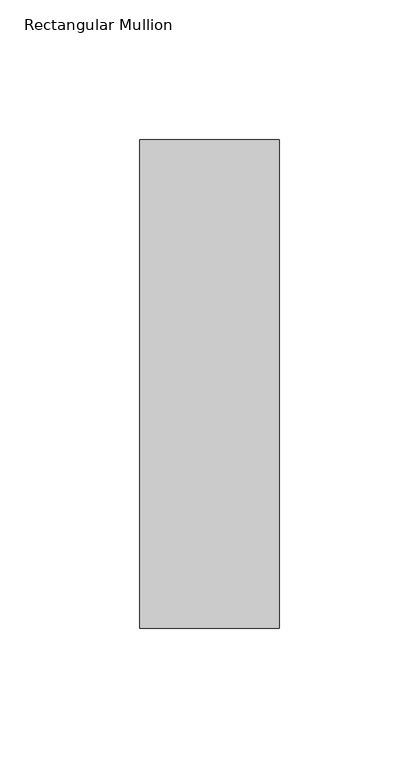
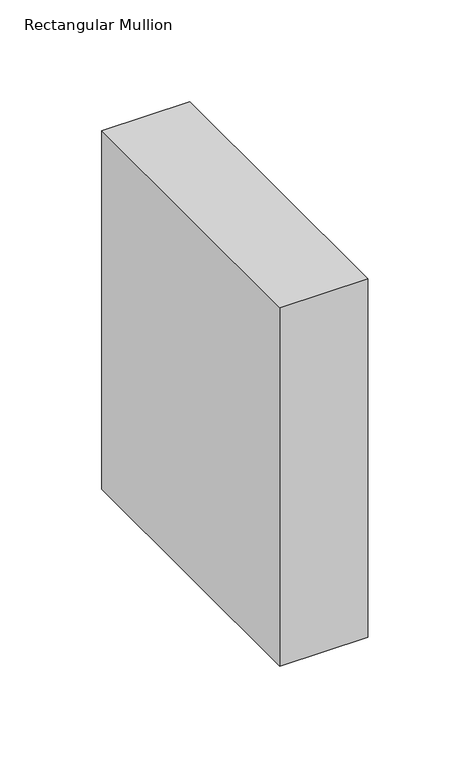
"""IFC4 building model written with IfcOpenShell, lengths in millimetres: member geometry, Rectangular Mullion : WWm-50x175-50mmOffset."""

import ifcopenshell
import ifcopenshell.guid

model = None  # the IFC model being written
_history = None  # IfcOwnerHistory: only IFC2X3 demands one
_inside = {}  # id of a spatial element -> (the spatial element, [elements in it])
_under = {}  # id of a project, library or spatial element -> (it, [spatial elements below it])
_declared = {}  # id of a project -> (the project, [libraries it declares])
_typed = {}  # id of a type object -> (the type object, [elements of that type])
_made_of = {}  # id of a material, layer set ... -> (it, [elements and type objects made of it])


def new_model(schema):
    """Start an empty IFC model of exactly this schema.

    Asked for "IFC4X3", IfcOpenShell would pick the latest addendum, in which some entities
    have other attributes; the version numbers below select the first issue.
    IFC2X3 requires an IfcOwnerHistory on every rooted entity: one is made here for all.
    """
    global model, _history
    if schema == "IFC4X3":
        model = ifcopenshell.file(schema_version=(4, 3, 0, 0))
    else:
        model = ifcopenshell.file(schema=schema)
    _inside.clear()
    _under.clear()
    _declared.clear()
    _typed.clear()
    _made_of.clear()
    _history = None
    if model.schema == "IFC2X3":
        org = make("IfcOrganization", Name="unknown")
        user = make(
            "IfcPersonAndOrganization",
            ThePerson=make("IfcPerson", FamilyName="unknown"),
            TheOrganization=org,
        )
        app = make(
            "IfcApplication",
            ApplicationDeveloper=org,
            Version="unknown",
            ApplicationFullName="unknown",
            ApplicationIdentifier="unknown",
        )
        _history = make(
            "IfcOwnerHistory",
            OwningUser=user,
            OwningApplication=app,
            ChangeAction="ADDED",
            CreationDate=0,
        )
    return model


def make(cls, **values):
    """One entity of the class cls with the attributes given. An attribute that is None is left unset."""
    return model.create_entity(
        cls, **{name: value for name, value in values.items() if value is not None}
    )


def rooted(cls, **values):
    """An entity with a GlobalId (a new one), such as an element, a storey or a relation."""
    return make(cls, GlobalId=ifcopenshell.guid.new(), OwnerHistory=_history, **values)


def si_unit(unit_type, name, prefix=None):
    """IfcSIUnit, for example si_unit("LENGTHUNIT", "METRE", prefix="MILLI")."""
    return make("IfcSIUnit", UnitType=unit_type, Prefix=prefix, Name=name)


def assignment(units):
    """IfcUnitAssignment: the units of a project."""
    return None if units is None else make("IfcUnitAssignment", Units=units)


def point(xyz):
    """IfcCartesianPoint."""
    return None if xyz is None else make("IfcCartesianPoint", Coordinates=xyz)


def direction(xyz):
    """IfcDirection."""
    return None if xyz is None else make("IfcDirection", DirectionRatios=xyz)


def frame(location, z_axis=None, x_axis=None):
    """IfcAxis2Placement3D, a coordinate frame: its origin and axes. An axis left out is left unset."""
    return make(
        "IfcAxis2Placement3D",
        Location=point(location),
        Axis=direction(z_axis),
        RefDirection=direction(x_axis),
    )


def origin():
    """The frame at (0, 0, 0) with its axes left unset."""
    return frame((0.0, 0.0, 0.0))


def place(relative_to, where):
    """IfcLocalPlacement: puts the frame where relative to a parent placement (None: the world)."""
    return make(
        "IfcLocalPlacement", PlacementRelTo=relative_to, RelativePlacement=where
    )


def context(
    kind, dimensions, precision=None, world=None, true_north=None, identifier=None
):
    """IfcGeometricRepresentationContext, for example the 3D "Model" context."""
    return make(
        "IfcGeometricRepresentationContext",
        ContextIdentifier=identifier,
        ContextType=kind,
        CoordinateSpaceDimension=dimensions,
        Precision=precision,
        WorldCoordinateSystem=world,
        TrueNorth=true_north,
    )


def project(units=None, contexts=None):
    """IfcProject with its units and contexts."""
    return rooted(
        "IfcProject",
        Name="project",
        RepresentationContexts=contexts,
        UnitsInContext=assignment(units),
    )


def spatial(cls, under=None, at=None, **own):
    """A site, building, storey or space (cls), placed at a placement, below another one or the project."""
    s = rooted(cls, ObjectPlacement=at, **own)
    if under is not None:
        _under.setdefault(under.id(), (under, []))[1].append(s)
    return s


def polyline(points):
    """IfcPolyline through the points."""
    return make("IfcPolyline", Points=[point(p) for p in points])


def outline(outer, holes=None, kind="AREA"):
    """IfcArbitraryClosedProfileDef: a profile drawn as a closed curve; with holes, ...WithVoids."""
    if holes is None:
        return make("IfcArbitraryClosedProfileDef", ProfileType=kind, OuterCurve=outer)
    return make(
        "IfcArbitraryProfileDefWithVoids",
        ProfileType=kind,
        OuterCurve=outer,
        InnerCurves=holes,
    )


def extrude(swept, where, along, depth):
    """IfcExtrudedAreaSolid: the profile swept, set in the frame where, extruded along a direction by depth."""
    return make(
        "IfcExtrudedAreaSolid",
        SweptArea=swept,
        Position=where,
        ExtrudedDirection=direction(along),
        Depth=depth,
    )


def shape(context_of_items, identifier, shape_type, items):
    """IfcShapeRepresentation: the items that make up one representation, for example the "Body"."""
    return make(
        "IfcShapeRepresentation",
        ContextOfItems=context_of_items,
        RepresentationIdentifier=identifier,
        RepresentationType=shape_type,
        Items=items,
    )


def source(mapping_origin, context_of_items, identifier, shape_type, items):
    """IfcRepresentationMap: a shape defined once, which mapped items show again and again."""
    return make(
        "IfcRepresentationMap",
        MappingOrigin=mapping_origin,
        MappedRepresentation=shape(context_of_items, identifier, shape_type, items),
    )


def transform(
    local_origin,
    x_axis=None,
    y_axis=None,
    z_axis=None,
    scale=None,
    scale2=None,
    scale3=None,
    uniform=True,
):
    """IfcCartesianTransformationOperator3D, or its non-uniform kind. x_axis, y_axis, z_axis: its Axis1, 2, 3."""
    if uniform:
        return make(
            "IfcCartesianTransformationOperator3D",
            Axis1=direction(x_axis),
            Axis2=direction(y_axis),
            LocalOrigin=point(local_origin),
            Scale=scale,
            Axis3=direction(z_axis),
        )
    return make(
        "IfcCartesianTransformationOperator3DnonUniform",
        Axis1=direction(x_axis),
        Axis2=direction(y_axis),
        LocalOrigin=point(local_origin),
        Scale=scale,
        Axis3=direction(z_axis),
        Scale2=scale2,
        Scale3=scale3,
    )


def mapped(mapping_source, mapping_target):
    """IfcMappedItem: shows the shape of a source again, moved by a transform."""
    return make(
        "IfcMappedItem", MappingSource=mapping_source, MappingTarget=mapping_target
    )


def made_of(thing, what):
    """Note that an element or type object is made of a material, layer set ...; save() writes the relation."""
    if what is not None:
        _made_of.setdefault(what.id(), (what, []))[1].append(thing)
    return thing


def element(
    cls,
    number,
    at=None,
    inside=None,
    cuts=None,
    type_object=None,
    material=None,
    context=None,
    identifier="Body",
    shape_type=None,
    held_by="IfcProductDefinitionShape",
    body=None,
    shapes=None,
    **own,
):
    """One element of the class cls, such as IfcWall. Its Tag is "e" and its number.

    at: its placement. inside: the storey or other place that contains it. cuts: it is an
    opening in that element (IfcRelVoidsElement). A single representation is given by context,
    identifier, shape_type and body (its items); several are given by shapes. held_by: the class
    of the entity that holds the representations. save() writes the other relations.
    """
    e = rooted(cls, Tag="e%d" % number, ObjectPlacement=at, **own)
    if body is not None:
        shapes = [shape(context, identifier, shape_type, body)]
    if shapes is not None:
        e.Representation = make(held_by, Representations=shapes)
    if inside is not None:
        _inside.setdefault(inside.id(), (inside, []))[1].append(e)
    if cuts is not None:
        rooted(
            "IfcRelVoidsElement", RelatingBuildingElement=cuts, RelatedOpeningElement=e
        )
    if type_object is not None:
        _typed.setdefault(type_object.id(), (type_object, []))[1].append(e)
    return made_of(e, material)


def aggregate(whole, parts):
    """IfcRelAggregates: a whole, such as a stair, and the parts it consists of."""
    return rooted("IfcRelAggregates", RelatingObject=whole, RelatedObjects=parts)


def save(model, path):
    """Write the relations noted so far, then the file.

    IfcRelAggregates (storeys below a building ...), IfcRelContainedInSpatialStructure (elements
    in a storey), IfcRelDefinesByType, IfcRelAssociatesMaterial and IfcRelDeclares: one each for
    every whole, place, type object, material and project.
    """
    for whole, parts in _under.values():
        aggregate(whole, parts)
    for where, things in _inside.values():
        rooted(
            "IfcRelContainedInSpatialStructure",
            RelatedElements=things,
            RelatingStructure=where,
        )
    for kind, things in _typed.values():
        rooted("IfcRelDefinesByType", RelatedObjects=things, RelatingType=kind)
    for what, things in _made_of.values():
        rooted("IfcRelAssociatesMaterial", RelatedObjects=things, RelatingMaterial=what)
    for by, libraries in _declared.values():
        rooted("IfcRelDeclares", RelatingContext=by, RelatedDefinitions=libraries)
    model.write(path)


def rectangular_mullion_eb0bb784(model_context):
    return source(origin(), model_context, "Body", "SweptSolid", [
        extrude(outline(polyline([(0.0, 87.5), (0.0, -87.5), (-50.0, -87.5), (-50.0, 87.5), (0.0, 87.5)])), frame((0.0, 0.0, -215.0), z_axis=(0.0, 0.0, 1.0), x_axis=(1.0, 0.0, 0.0)), (0.0, 0.0, 1.0), 215.0),
    ])


if __name__ == "__main__":
    model = new_model("IFC4")
    model_context = context("Model", 3, world=origin())
    ifc_project = project(units=[si_unit("LENGTHUNIT", "METRE", prefix="MILLI")], contexts=[model_context])
    site = spatial("IfcSite", under=ifc_project)
    building = spatial("IfcBuilding", under=site)
    placement = place(None, origin())
    rectangular_mullion_shape = rectangular_mullion_eb0bb784(model_context)
    element("IfcMember", 1, ObjectType="Rectangular Mullion : WWm-50x175-50mmOffset", at=placement, inside=building, context=model_context, shape_type="MappedRepresentation", body=[
        mapped(rectangular_mullion_shape, transform((0.0, 0.0, 0.0), x_axis=(1.0, 0.0, 0.0), y_axis=(0.0, 1.0, 0.0), z_axis=(0.0, 0.0, 1.0))),
    ])
    save(model, "model.ifc")

# Revit data of these elements
# Type "Rectangular Mullion : WWm-50x175-50mmOffset"
#   built-in parameter 1007304 = 0.574147 (stored number, unit not read)
#   built-in parameter 1007301 = 0.082021 (stored number, unit not read)
#   built-in parameter 1007300 = 0.082021 (stored number, unit not read)
# Element 1 (IfcMember, "Rectangular Mullion : WWm-50x175-50mmOffset")
#   Materials on its faces: "WW-EC-RGB-Mullion"
# Materials
#   "WW-EC-RGB-Mullion": class "Generic", colour RGB 255 255 255, transparency 0, Comments = "If region requests black mullions, switch asset color to RGB 25-25-25", Description = "Generic Color", Cost = 0
